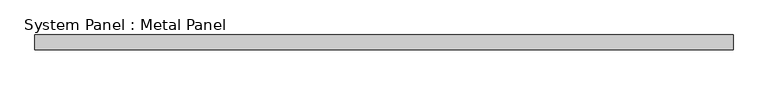
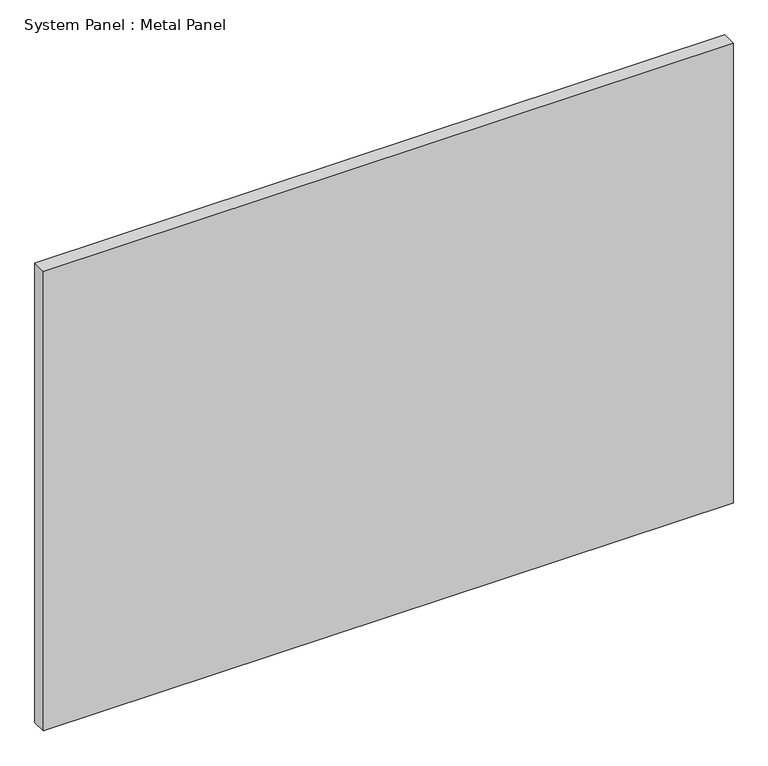
"""IFC4 building model written with IfcOpenShell, lengths in millimetres: plate geometry, System Panel : Metal Panel."""

import ifcopenshell
import ifcopenshell.guid

model = None  # the IFC model being written
_history = None  # IfcOwnerHistory: only IFC2X3 demands one
_inside = {}  # id of a spatial element -> (the spatial element, [elements in it])
_under = {}  # id of a project, library or spatial element -> (it, [spatial elements below it])
_declared = {}  # id of a project -> (the project, [libraries it declares])
_typed = {}  # id of a type object -> (the type object, [elements of that type])
_made_of = {}  # id of a material, layer set ... -> (it, [elements and type objects made of it])


def new_model(schema):
    """Start an empty IFC model of exactly this schema.

    Asked for "IFC4X3", IfcOpenShell would pick the latest addendum, in which some entities
    have other attributes; the version numbers below select the first issue.
    IFC2X3 requires an IfcOwnerHistory on every rooted entity: one is made here for all.
    """
    global model, _history
    if schema == "IFC4X3":
        model = ifcopenshell.file(schema_version=(4, 3, 0, 0))
    else:
        model = ifcopenshell.file(schema=schema)
    _inside.clear()
    _under.clear()
    _declared.clear()
    _typed.clear()
    _made_of.clear()
    _history = None
    if model.schema == "IFC2X3":
        org = make("IfcOrganization", Name="unknown")
        user = make(
            "IfcPersonAndOrganization",
            ThePerson=make("IfcPerson", FamilyName="unknown"),
            TheOrganization=org,
        )
        app = make(
            "IfcApplication",
            ApplicationDeveloper=org,
            Version="unknown",
            ApplicationFullName="unknown",
            ApplicationIdentifier="unknown",
        )
        _history = make(
            "IfcOwnerHistory",
            OwningUser=user,
            OwningApplication=app,
            ChangeAction="ADDED",
            CreationDate=0,
        )
    return model


def make(cls, **values):
    """One entity of the class cls with the attributes given. An attribute that is None is left unset."""
    return model.create_entity(
        cls, **{name: value for name, value in values.items() if value is not None}
    )


def rooted(cls, **values):
    """An entity with a GlobalId (a new one), such as an element, a storey or a relation."""
    return make(cls, GlobalId=ifcopenshell.guid.new(), OwnerHistory=_history, **values)


def si_unit(unit_type, name, prefix=None):
    """IfcSIUnit, for example si_unit("LENGTHUNIT", "METRE", prefix="MILLI")."""
    return make("IfcSIUnit", UnitType=unit_type, Prefix=prefix, Name=name)


def assignment(units):
    """IfcUnitAssignment: the units of a project."""
    return None if units is None else make("IfcUnitAssignment", Units=units)


def point(xyz):
    """IfcCartesianPoint."""
    return None if xyz is None else make("IfcCartesianPoint", Coordinates=xyz)


def direction(xyz):
    """IfcDirection."""
    return None if xyz is None else make("IfcDirection", DirectionRatios=xyz)


def frame(location, z_axis=None, x_axis=None):
    """IfcAxis2Placement3D, a coordinate frame: its origin and axes. An axis left out is left unset."""
    return make(
        "IfcAxis2Placement3D",
        Location=point(location),
        Axis=direction(z_axis),
        RefDirection=direction(x_axis),
    )


def origin():
    """The frame at (0, 0, 0) with its axes left unset."""
    return frame((0.0, 0.0, 0.0))


def origin_with_axes():
    """The frame at (0, 0, 0) with the z axis (0, 0, 1) and the x axis (1, 0, 0) written out."""
    return frame((0.0, 0.0, 0.0), z_axis=(0.0, 0.0, 1.0), x_axis=(1.0, 0.0, 0.0))


def place(relative_to, where):
    """IfcLocalPlacement: puts the frame where relative to a parent placement (None: the world)."""
    return make(
        "IfcLocalPlacement", PlacementRelTo=relative_to, RelativePlacement=where
    )


def context(
    kind, dimensions, precision=None, world=None, true_north=None, identifier=None
):
    """IfcGeometricRepresentationContext, for example the 3D "Model" context."""
    return make(
        "IfcGeometricRepresentationContext",
        ContextIdentifier=identifier,
        ContextType=kind,
        CoordinateSpaceDimension=dimensions,
        Precision=precision,
        WorldCoordinateSystem=world,
        TrueNorth=true_north,
    )


def project(units=None, contexts=None):
    """IfcProject with its units and contexts."""
    return rooted(
        "IfcProject",
        Name="project",
        RepresentationContexts=contexts,
        UnitsInContext=assignment(units),
    )


def spatial(cls, under=None, at=None, **own):
    """A site, building, storey or space (cls), placed at a placement, below another one or the project."""
    s = rooted(cls, ObjectPlacement=at, **own)
    if under is not None:
        _under.setdefault(under.id(), (under, []))[1].append(s)
    return s


def polyline(points):
    """IfcPolyline through the points."""
    return make("IfcPolyline", Points=[point(p) for p in points])


def outline(outer, holes=None, kind="AREA"):
    """IfcArbitraryClosedProfileDef: a profile drawn as a closed curve; with holes, ...WithVoids."""
    if holes is None:
        return make("IfcArbitraryClosedProfileDef", ProfileType=kind, OuterCurve=outer)
    return make(
        "IfcArbitraryProfileDefWithVoids",
        ProfileType=kind,
        OuterCurve=outer,
        InnerCurves=holes,
    )


def extrude(swept, where, along, depth):
    """IfcExtrudedAreaSolid: the profile swept, set in the frame where, extruded along a direction by depth."""
    return make(
        "IfcExtrudedAreaSolid",
        SweptArea=swept,
        Position=where,
        ExtrudedDirection=direction(along),
        Depth=depth,
    )


def shape(context_of_items, identifier, shape_type, items):
    """IfcShapeRepresentation: the items that make up one representation, for example the "Body"."""
    return make(
        "IfcShapeRepresentation",
        ContextOfItems=context_of_items,
        RepresentationIdentifier=identifier,
        RepresentationType=shape_type,
        Items=items,
    )


def source(mapping_origin, context_of_items, identifier, shape_type, items):
    """IfcRepresentationMap: a shape defined once, which mapped items show again and again."""
    return make(
        "IfcRepresentationMap",
        MappingOrigin=mapping_origin,
        MappedRepresentation=shape(context_of_items, identifier, shape_type, items),
    )


def transform(
    local_origin,
    x_axis=None,
    y_axis=None,
    z_axis=None,
    scale=None,
    scale2=None,
    scale3=None,
    uniform=True,
):
    """IfcCartesianTransformationOperator3D, or its non-uniform kind. x_axis, y_axis, z_axis: its Axis1, 2, 3."""
    if uniform:
        return make(
            "IfcCartesianTransformationOperator3D",
            Axis1=direction(x_axis),
            Axis2=direction(y_axis),
            LocalOrigin=point(local_origin),
            Scale=scale,
            Axis3=direction(z_axis),
        )
    return make(
        "IfcCartesianTransformationOperator3DnonUniform",
        Axis1=direction(x_axis),
        Axis2=direction(y_axis),
        LocalOrigin=point(local_origin),
        Scale=scale,
        Axis3=direction(z_axis),
        Scale2=scale2,
        Scale3=scale3,
    )


def mapped(mapping_source, mapping_target):
    """IfcMappedItem: shows the shape of a source again, moved by a transform."""
    return make(
        "IfcMappedItem", MappingSource=mapping_source, MappingTarget=mapping_target
    )


def made_of(thing, what):
    """Note that an element or type object is made of a material, layer set ...; save() writes the relation."""
    if what is not None:
        _made_of.setdefault(what.id(), (what, []))[1].append(thing)
    return thing


def element(
    cls,
    number,
    at=None,
    inside=None,
    cuts=None,
    type_object=None,
    material=None,
    context=None,
    identifier="Body",
    shape_type=None,
    held_by="IfcProductDefinitionShape",
    body=None,
    shapes=None,
    **own,
):
    """One element of the class cls, such as IfcWall. Its Tag is "e" and its number.

    at: its placement. inside: the storey or other place that contains it. cuts: it is an
    opening in that element (IfcRelVoidsElement). A single representation is given by context,
    identifier, shape_type and body (its items); several are given by shapes. held_by: the class
    of the entity that holds the representations. save() writes the other relations.
    """
    e = rooted(cls, Tag="e%d" % number, ObjectPlacement=at, **own)
    if body is not None:
        shapes = [shape(context, identifier, shape_type, body)]
    if shapes is not None:
        e.Representation = make(held_by, Representations=shapes)
    if inside is not None:
        _inside.setdefault(inside.id(), (inside, []))[1].append(e)
    if cuts is not None:
        rooted(
            "IfcRelVoidsElement", RelatingBuildingElement=cuts, RelatedOpeningElement=e
        )
    if type_object is not None:
        _typed.setdefault(type_object.id(), (type_object, []))[1].append(e)
    return made_of(e, material)


def aggregate(whole, parts):
    """IfcRelAggregates: a whole, such as a stair, and the parts it consists of."""
    return rooted("IfcRelAggregates", RelatingObject=whole, RelatedObjects=parts)


def save(model, path):
    """Write the relations noted so far, then the file.

    IfcRelAggregates (storeys below a building ...), IfcRelContainedInSpatialStructure (elements
    in a storey), IfcRelDefinesByType, IfcRelAssociatesMaterial and IfcRelDeclares: one each for
    every whole, place, type object, material and project.
    """
    for whole, parts in _under.values():
        aggregate(whole, parts)
    for where, things in _inside.values():
        rooted(
            "IfcRelContainedInSpatialStructure",
            RelatedElements=things,
            RelatingStructure=where,
        )
    for kind, things in _typed.values():
        rooted("IfcRelDefinesByType", RelatedObjects=things, RelatingType=kind)
    for what, things in _made_of.values():
        rooted("IfcRelAssociatesMaterial", RelatedObjects=things, RelatingMaterial=what)
    for by, libraries in _declared.values():
        rooted("IfcRelDeclares", RelatingContext=by, RelatedDefinitions=libraries)
    model.write(path)


def system_panel_metal_panel_dcd9a435(model_context):
    return source(origin(), model_context, "Body", "SweptSolid", [
        extrude(outline(polyline([(603.7494819, 19.05), (-603.7494819, 19.05), (-603.7494819, 44.45), (603.7494819, 44.45), (603.7494819, 19.05)])), origin_with_axes(), (0.0, 0.0, 1.0), 850.9),
    ])


if __name__ == "__main__":
    model = new_model("IFC4")
    model_context = context("Model", 3, world=origin())
    ifc_project = project(units=[si_unit("LENGTHUNIT", "METRE", prefix="MILLI")], contexts=[model_context])
    site = spatial("IfcSite", under=ifc_project)
    building = spatial("IfcBuilding", under=site)
    placement = place(None, origin())
    system_panel_metal_panel_shape = system_panel_metal_panel_dcd9a435(model_context)
    element("IfcPlate", 1, ObjectType="System Panel : Metal Panel", at=placement, inside=building, context=model_context, shape_type="MappedRepresentation", body=[
        mapped(system_panel_metal_panel_shape, transform((0.0, 0.0, 0.0), x_axis=(1.0, 0.0, 0.0), y_axis=(0.0, 1.0, 0.0), z_axis=(0.0, 0.0, 1.0))),
    ])
    save(model, "model.ifc")

# Revit data of these elements
# Element 1 (IfcPlate, "System Panel : Metal Panel")
#   Materials on its faces: "Aluminum"
# Materials
#   "Aluminum": class "Metal", colour RGB 247 247 247, transparency 0, Description = "Aluminum 6061", Cost = 0
